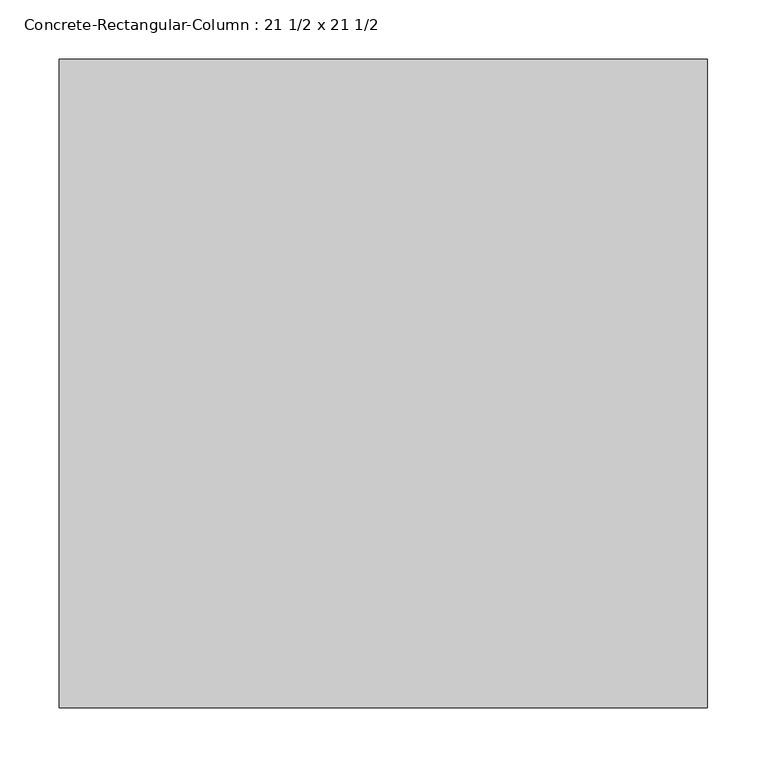
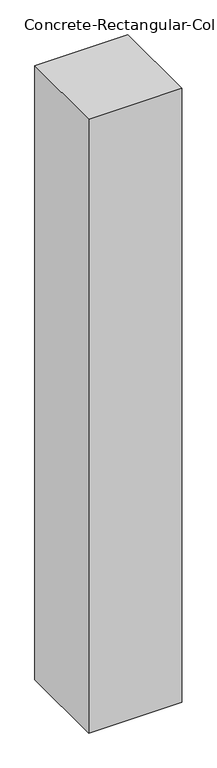
"""IFC4 building model written with IfcOpenShell, lengths in millimetres: column geometry, Concrete-Rectangular-Column : 21 1/2 x 21 1/2."""

import ifcopenshell
import ifcopenshell.guid

model = None  # the IFC model being written
_history = None  # IfcOwnerHistory: only IFC2X3 demands one
_inside = {}  # id of a spatial element -> (the spatial element, [elements in it])
_under = {}  # id of a project, library or spatial element -> (it, [spatial elements below it])
_declared = {}  # id of a project -> (the project, [libraries it declares])
_typed = {}  # id of a type object -> (the type object, [elements of that type])
_made_of = {}  # id of a material, layer set ... -> (it, [elements and type objects made of it])


def new_model(schema):
    """Start an empty IFC model of exactly this schema.

    Asked for "IFC4X3", IfcOpenShell would pick the latest addendum, in which some entities
    have other attributes; the version numbers below select the first issue.
    IFC2X3 requires an IfcOwnerHistory on every rooted entity: one is made here for all.
    """
    global model, _history
    if schema == "IFC4X3":
        model = ifcopenshell.file(schema_version=(4, 3, 0, 0))
    else:
        model = ifcopenshell.file(schema=schema)
    _inside.clear()
    _under.clear()
    _declared.clear()
    _typed.clear()
    _made_of.clear()
    _history = None
    if model.schema == "IFC2X3":
        org = make("IfcOrganization", Name="unknown")
        user = make(
            "IfcPersonAndOrganization",
            ThePerson=make("IfcPerson", FamilyName="unknown"),
            TheOrganization=org,
        )
        app = make(
            "IfcApplication",
            ApplicationDeveloper=org,
            Version="unknown",
            ApplicationFullName="unknown",
            ApplicationIdentifier="unknown",
        )
        _history = make(
            "IfcOwnerHistory",
            OwningUser=user,
            OwningApplication=app,
            ChangeAction="ADDED",
            CreationDate=0,
        )
    return model


def make(cls, **values):
    """One entity of the class cls with the attributes given. An attribute that is None is left unset."""
    return model.create_entity(
        cls, **{name: value for name, value in values.items() if value is not None}
    )


def rooted(cls, **values):
    """An entity with a GlobalId (a new one), such as an element, a storey or a relation."""
    return make(cls, GlobalId=ifcopenshell.guid.new(), OwnerHistory=_history, **values)


def si_unit(unit_type, name, prefix=None):
    """IfcSIUnit, for example si_unit("LENGTHUNIT", "METRE", prefix="MILLI")."""
    return make("IfcSIUnit", UnitType=unit_type, Prefix=prefix, Name=name)


def assignment(units):
    """IfcUnitAssignment: the units of a project."""
    return None if units is None else make("IfcUnitAssignment", Units=units)


def point(xyz):
    """IfcCartesianPoint."""
    return None if xyz is None else make("IfcCartesianPoint", Coordinates=xyz)


def direction(xyz):
    """IfcDirection."""
    return None if xyz is None else make("IfcDirection", DirectionRatios=xyz)


def frame(location, z_axis=None, x_axis=None):
    """IfcAxis2Placement3D, a coordinate frame: its origin and axes. An axis left out is left unset."""
    return make(
        "IfcAxis2Placement3D",
        Location=point(location),
        Axis=direction(z_axis),
        RefDirection=direction(x_axis),
    )


def origin():
    """The frame at (0, 0, 0) with its axes left unset."""
    return frame((0.0, 0.0, 0.0))


def origin_with_axes():
    """The frame at (0, 0, 0) with the z axis (0, 0, 1) and the x axis (1, 0, 0) written out."""
    return frame((0.0, 0.0, 0.0), z_axis=(0.0, 0.0, 1.0), x_axis=(1.0, 0.0, 0.0))


def place(relative_to, where):
    """IfcLocalPlacement: puts the frame where relative to a parent placement (None: the world)."""
    return make(
        "IfcLocalPlacement", PlacementRelTo=relative_to, RelativePlacement=where
    )


def context(
    kind, dimensions, precision=None, world=None, true_north=None, identifier=None
):
    """IfcGeometricRepresentationContext, for example the 3D "Model" context."""
    return make(
        "IfcGeometricRepresentationContext",
        ContextIdentifier=identifier,
        ContextType=kind,
        CoordinateSpaceDimension=dimensions,
        Precision=precision,
        WorldCoordinateSystem=world,
        TrueNorth=true_north,
    )


def project(units=None, contexts=None):
    """IfcProject with its units and contexts."""
    return rooted(
        "IfcProject",
        Name="project",
        RepresentationContexts=contexts,
        UnitsInContext=assignment(units),
    )


def spatial(cls, under=None, at=None, **own):
    """A site, building, storey or space (cls), placed at a placement, below another one or the project."""
    s = rooted(cls, ObjectPlacement=at, **own)
    if under is not None:
        _under.setdefault(under.id(), (under, []))[1].append(s)
    return s


def polyline(points):
    """IfcPolyline through the points."""
    return make("IfcPolyline", Points=[point(p) for p in points])


def outline(outer, holes=None, kind="AREA"):
    """IfcArbitraryClosedProfileDef: a profile drawn as a closed curve; with holes, ...WithVoids."""
    if holes is None:
        return make("IfcArbitraryClosedProfileDef", ProfileType=kind, OuterCurve=outer)
    return make(
        "IfcArbitraryProfileDefWithVoids",
        ProfileType=kind,
        OuterCurve=outer,
        InnerCurves=holes,
    )


def extrude(swept, where, along, depth):
    """IfcExtrudedAreaSolid: the profile swept, set in the frame where, extruded along a direction by depth."""
    return make(
        "IfcExtrudedAreaSolid",
        SweptArea=swept,
        Position=where,
        ExtrudedDirection=direction(along),
        Depth=depth,
    )


def shape(context_of_items, identifier, shape_type, items):
    """IfcShapeRepresentation: the items that make up one representation, for example the "Body"."""
    return make(
        "IfcShapeRepresentation",
        ContextOfItems=context_of_items,
        RepresentationIdentifier=identifier,
        RepresentationType=shape_type,
        Items=items,
    )


def source(mapping_origin, context_of_items, identifier, shape_type, items):
    """IfcRepresentationMap: a shape defined once, which mapped items show again and again."""
    return make(
        "IfcRepresentationMap",
        MappingOrigin=mapping_origin,
        MappedRepresentation=shape(context_of_items, identifier, shape_type, items),
    )


def transform(
    local_origin,
    x_axis=None,
    y_axis=None,
    z_axis=None,
    scale=None,
    scale2=None,
    scale3=None,
    uniform=True,
):
    """IfcCartesianTransformationOperator3D, or its non-uniform kind. x_axis, y_axis, z_axis: its Axis1, 2, 3."""
    if uniform:
        return make(
            "IfcCartesianTransformationOperator3D",
            Axis1=direction(x_axis),
            Axis2=direction(y_axis),
            LocalOrigin=point(local_origin),
            Scale=scale,
            Axis3=direction(z_axis),
        )
    return make(
        "IfcCartesianTransformationOperator3DnonUniform",
        Axis1=direction(x_axis),
        Axis2=direction(y_axis),
        LocalOrigin=point(local_origin),
        Scale=scale,
        Axis3=direction(z_axis),
        Scale2=scale2,
        Scale3=scale3,
    )


def mapped(mapping_source, mapping_target):
    """IfcMappedItem: shows the shape of a source again, moved by a transform."""
    return make(
        "IfcMappedItem", MappingSource=mapping_source, MappingTarget=mapping_target
    )


def made_of(thing, what):
    """Note that an element or type object is made of a material, layer set ...; save() writes the relation."""
    if what is not None:
        _made_of.setdefault(what.id(), (what, []))[1].append(thing)
    return thing


def element(
    cls,
    number,
    at=None,
    inside=None,
    cuts=None,
    type_object=None,
    material=None,
    context=None,
    identifier="Body",
    shape_type=None,
    held_by="IfcProductDefinitionShape",
    body=None,
    shapes=None,
    **own,
):
    """One element of the class cls, such as IfcWall. Its Tag is "e" and its number.

    at: its placement. inside: the storey or other place that contains it. cuts: it is an
    opening in that element (IfcRelVoidsElement). A single representation is given by context,
    identifier, shape_type and body (its items); several are given by shapes. held_by: the class
    of the entity that holds the representations. save() writes the other relations.
    """
    e = rooted(cls, Tag="e%d" % number, ObjectPlacement=at, **own)
    if body is not None:
        shapes = [shape(context, identifier, shape_type, body)]
    if shapes is not None:
        e.Representation = make(held_by, Representations=shapes)
    if inside is not None:
        _inside.setdefault(inside.id(), (inside, []))[1].append(e)
    if cuts is not None:
        rooted(
            "IfcRelVoidsElement", RelatingBuildingElement=cuts, RelatedOpeningElement=e
        )
    if type_object is not None:
        _typed.setdefault(type_object.id(), (type_object, []))[1].append(e)
    return made_of(e, material)


def aggregate(whole, parts):
    """IfcRelAggregates: a whole, such as a stair, and the parts it consists of."""
    return rooted("IfcRelAggregates", RelatingObject=whole, RelatedObjects=parts)


def save(model, path):
    """Write the relations noted so far, then the file.

    IfcRelAggregates (storeys below a building ...), IfcRelContainedInSpatialStructure (elements
    in a storey), IfcRelDefinesByType, IfcRelAssociatesMaterial and IfcRelDeclares: one each for
    every whole, place, type object, material and project.
    """
    for whole, parts in _under.values():
        aggregate(whole, parts)
    for where, things in _inside.values():
        rooted(
            "IfcRelContainedInSpatialStructure",
            RelatedElements=things,
            RelatingStructure=where,
        )
    for kind, things in _typed.values():
        rooted("IfcRelDefinesByType", RelatedObjects=things, RelatingType=kind)
    for what, things in _made_of.values():
        rooted("IfcRelAssociatesMaterial", RelatedObjects=things, RelatingMaterial=what)
    for by, libraries in _declared.values():
        rooted("IfcRelDeclares", RelatingContext=by, RelatedDefinitions=libraries)
    model.write(path)


def concrete_rectangular_column_21_1_2_x_21_1_2_5e8797fa(model_context):
    return source(origin(), model_context, "Body", "SweptSolid", [
        extrude(outline(polyline([(273.05, -273.05), (-273.05, -273.05), (-273.05, 273.05), (273.05, 273.05), (273.05, -273.05)])), origin_with_axes(), (0.0, 0.0, 1.0), 3810.0),
    ])


if __name__ == "__main__":
    model = new_model("IFC4")
    model_context = context("Model", 3, world=origin())
    ifc_project = project(units=[si_unit("LENGTHUNIT", "METRE", prefix="MILLI")], contexts=[model_context])
    site = spatial("IfcSite", under=ifc_project)
    building = spatial("IfcBuilding", under=site)
    placement = place(None, origin())
    concrete_rectangular_column_21_1_2_x_21_1_2_shape = concrete_rectangular_column_21_1_2_x_21_1_2_5e8797fa(model_context)
    element("IfcColumn", 1, ObjectType="Concrete-Rectangular-Column : 21 1/2 x 21 1/2", at=placement, inside=building, context=model_context, shape_type="MappedRepresentation", body=[
        mapped(concrete_rectangular_column_21_1_2_x_21_1_2_shape, transform((0.0, 0.0, 0.0), x_axis=(1.0, 0.0, 0.0), y_axis=(0.0, 1.0, 0.0), z_axis=(0.0, 0.0, 1.0))),
    ])
    save(model, "model.ifc")

# Revit data of these elements
# Type "Concrete-Rectangular-Column : 21 1/2 x 21 1/2"
#   Assembly Code = "B10"
#   b = 546.1 mm
#   h = 546.1 mm
#   Structural Material [instance default] = Concrete - Cast-in-Place Concrete
# Element 1 (IfcColumn, "Concrete-Rectangular-Column : 21 1/2 x 21 1/2")
#   Materials on its faces: "Concrete - Cast-in-Place Concrete"
# Materials
#   "Concrete - Cast-in-Place Concrete": class "Concrete", colour RGB 192 192 192, transparency 0
